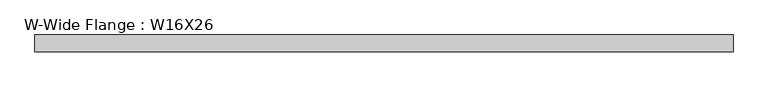
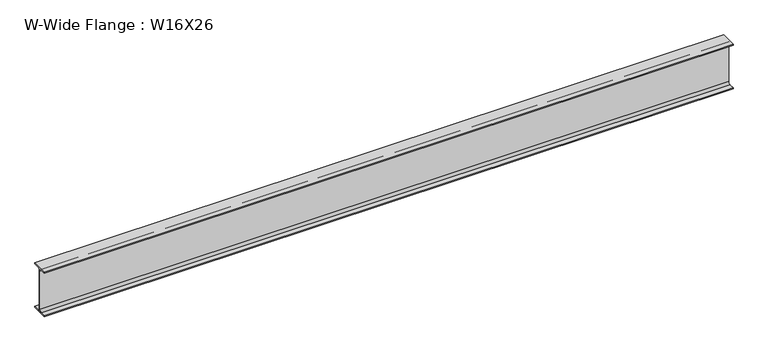
"""IFC4 building model written with IfcOpenShell, lengths in millimetres: beam geometry, W-Wide Flange : W16X26."""

from ifc_helpers import new_model, si_unit, point, frame, frame_2d, origin, place, context, project, spatial, polyline, circle_curve, trimmed, segment, composite_curve, outline, extrude, source, transform, mapped, element, save


def w_wide_flange_w16x26_e0fc420c(model_context):
    return source(origin(), model_context, "Body", "SweptSolid", [
        extrude(outline(composite_curve([segment(polyline([(69.85, -190.627), (69.85, -199.39), (-69.85, -199.39), (-69.85, -190.627), (-21.3995, -190.627)]), True, "CONTINUOUS"), segment(trimmed(circle_curve(frame_2d((-21.3995, -172.4025)), 18.2245), [point((-21.3995, -190.627))], [point((-3.175, -172.4025))], True, "CARTESIAN"), True, "CONTINUOUS"), segment(polyline([(-3.175, -172.4025), (-3.175, 172.4025)]), True, "CONTINUOUS"), segment(trimmed(circle_curve(frame_2d((-21.3995, 172.4025)), 18.2245), [point((-3.175, 172.4025))], [point((-21.3995, 190.627))], True, "CARTESIAN"), True, "CONTINUOUS"), segment(polyline([(-21.3995, 190.627), (-69.85, 190.627), (-69.85, 199.39), (69.85, 199.39), (69.85, 190.627), (21.3995, 190.627)]), True, "CONTINUOUS"), segment(trimmed(circle_curve(frame_2d((21.3995, 172.4025)), 18.2245), [point((21.3995, 190.627))], [point((3.175, 172.4025))], True, "CARTESIAN"), True, "CONTINUOUS"), segment(polyline([(3.175, 172.4025), (3.175, -172.4025)]), True, "CONTINUOUS"), segment(trimmed(circle_curve(frame_2d((21.3995, -172.4025)), 18.2245), [point((3.175, -172.4025))], [point((21.3995, -190.627))], True, "CARTESIAN"), True, "CONTINUOUS"), segment(polyline([(21.3995, -190.627), (69.85, -190.627)]), True, "CONTINUOUS")], self_intersect=False)), frame((-2921.0, 0.0, 0.0), z_axis=(1.0, 0.0, 0.0), x_axis=(0.0, 1.0, 0.0)), (0.0, 0.0, 1.0), 5842.0),
    ])


if __name__ == "__main__":
    model = new_model("IFC4")
    model_context = context("Model", 3, world=origin())
    ifc_project = project(units=[si_unit("LENGTHUNIT", "METRE", prefix="MILLI")], contexts=[model_context])
    site = spatial("IfcSite", under=ifc_project)
    building = spatial("IfcBuilding", under=site)
    placement = place(None, origin())
    w_wide_flange_w16x26_shape = w_wide_flange_w16x26_e0fc420c(model_context)
    element("IfcBeam", 1, ObjectType="W-Wide Flange : W16X26", at=placement, inside=building, context=model_context, shape_type="MappedRepresentation", body=[
        mapped(w_wide_flange_w16x26_shape, transform((0.0, 0.0, 0.0), x_axis=(1.0, 0.0, 0.0), y_axis=(0.0, 1.0, 0.0), z_axis=(0.0, 0.0, 1.0))),
    ])
    save(model, "model.ifc")

# Revit data of these elements
# Type "W-Wide Flange : W16X26"
#   Assembly Code = "B10"
#   W = 26
#   Length [instance default] = 5' - 0"
#   bf = 0' - 5 1/2"
#   d = 1' - 3.7"
#   k = 0' - 1 1/16"
#   k2 = 0' - 0.7175"
#   tf = 0' - 0.345"
#   tw = 0' - 0 1/4"
#   A = 0.0533333 SF
#   Structural Material [instance default] = Steel ASTM A992
# Element 1 (IfcBeam, "W-Wide Flange : W16X26")
#   Structural Material = Steel ASTM A36
#   Materials on its faces: "Steel ASTM A36"
# Materials
#   "Steel ASTM A992": class "Metal", colour RGB 199 199 199, transparency 0, Description = "Structural steel 50ksi", Cost = 0
#   "Steel ASTM A36": class "Metal", colour RGB 199 199 199, transparency 0, Description = "Structural steel, ASTM A36 Grade B, mill finish", Cost = 0
